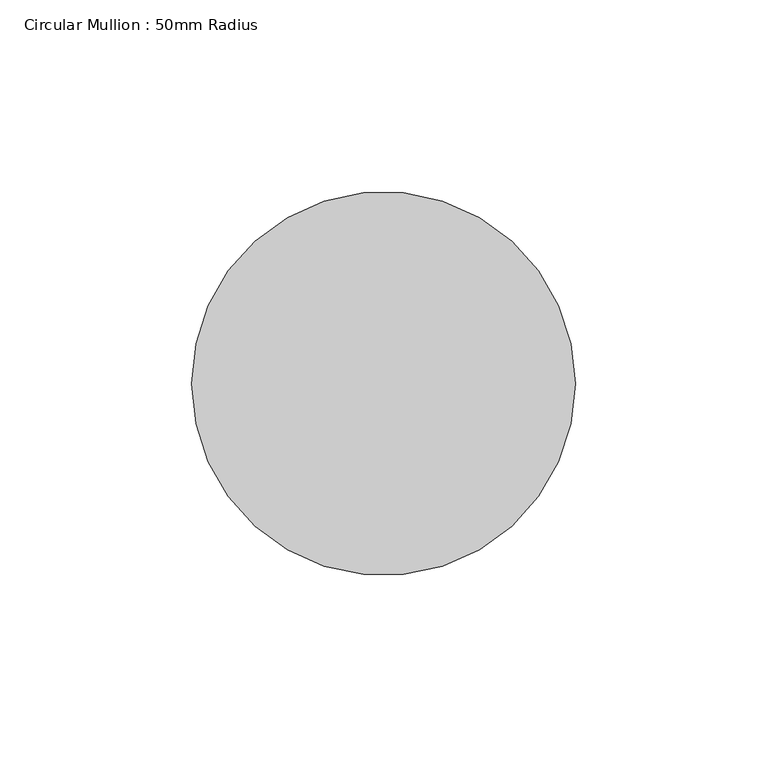
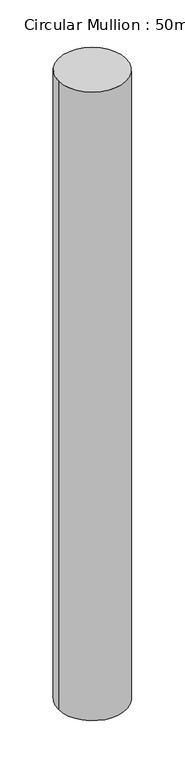
"""IFC4 building model written with IfcOpenShell, lengths in millimetres: member geometry, Circular Mullion : 50mm Radius."""

from ifc_helpers import new_model, si_unit, point, frame, origin, origin_2d, place, context, project, spatial, circle_curve, trimmed, segment, composite_curve, outline, extrude, source, transform, mapped, element, save


def circular_mullion_50mm_radius_d09b9a70(model_context):
    return source(origin(), model_context, "Body", "SweptSolid", [
        extrude(outline(composite_curve([segment(trimmed(circle_curve(origin_2d(), 50.0), [point((50.0, 0.0))], [point((-50.0, 0.0))], False, "CARTESIAN"), True, "CONTINUOUS"), segment(trimmed(circle_curve(origin_2d(), 50.0), [point((-50.0, 0.0))], [point((50.0, 0.0))], False, "CARTESIAN"), True, "CONTINUOUS")], self_intersect=False)), frame((0.0, 0.0, -981.2080075), z_axis=(0.0, 0.0, 1.0), x_axis=(1.0, 0.0, 0.0)), (0.0, 0.0, 1.0), 981.2080075),
    ])


if __name__ == "__main__":
    model = new_model("IFC4")
    model_context = context("Model", 3, world=origin())
    ifc_project = project(units=[si_unit("LENGTHUNIT", "METRE", prefix="MILLI")], contexts=[model_context])
    site = spatial("IfcSite", under=ifc_project)
    building = spatial("IfcBuilding", under=site)
    placement = place(None, origin())
    circular_mullion_50mm_radius_shape = circular_mullion_50mm_radius_d09b9a70(model_context)
    element("IfcMember", 1, ObjectType="Circular Mullion : 50mm Radius", at=placement, inside=building, context=model_context, shape_type="MappedRepresentation", body=[
        mapped(circular_mullion_50mm_radius_shape, transform((0.0, 0.0, 0.0), x_axis=(1.0, 0.0, 0.0), y_axis=(0.0, 1.0, 0.0), z_axis=(0.0, 0.0, 1.0))),
    ])
    save(model, "model.ifc")

# Revit data of these elements
# Type "Circular Mullion : 50mm Radius"
#   built-in parameter 1007350 = 0.164042 (stored number, unit not read)
# Element 1 (IfcMember, "Circular Mullion : 50mm Radius")
#   Materials on its faces: "Aluminium"
# Materials
#   "Aluminium": class "Metal", colour RGB 247 247 247, transparency 0, Description = "Aluminium 6061", Cost = 0
